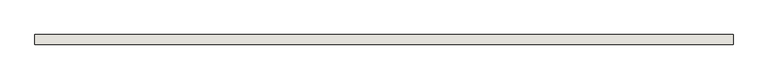
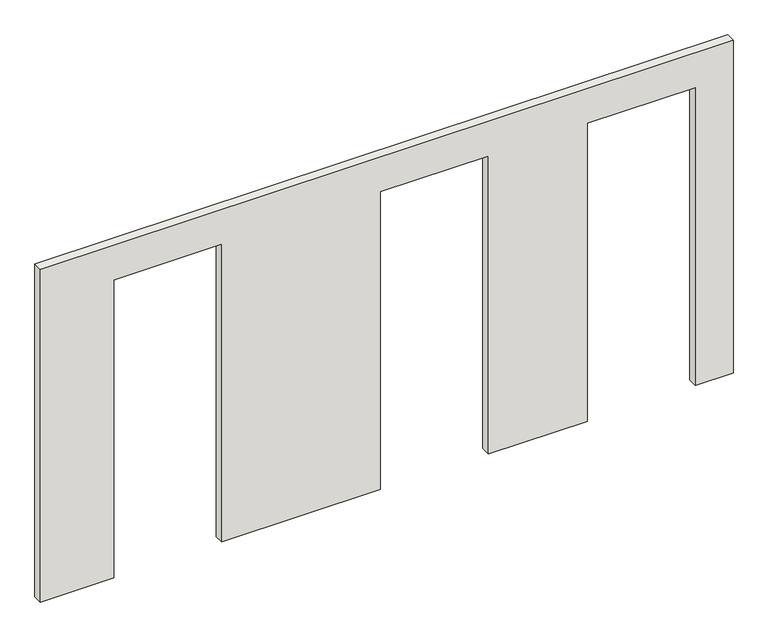
"""IFC4 building model written with IfcOpenShell, lengths in millimetres: wall geometry, 0_3d."""

import ifcopenshell
import ifcopenshell.guid

model = None  # the IFC model being written
_history = None  # IfcOwnerHistory: only IFC2X3 demands one
_inside = {}  # id of a spatial element -> (the spatial element, [elements in it])
_under = {}  # id of a project, library or spatial element -> (it, [spatial elements below it])
_declared = {}  # id of a project -> (the project, [libraries it declares])
_typed = {}  # id of a type object -> (the type object, [elements of that type])
_made_of = {}  # id of a material, layer set ... -> (it, [elements and type objects made of it])


def new_model(schema):
    """Start an empty IFC model of exactly this schema.

    Asked for "IFC4X3", IfcOpenShell would pick the latest addendum, in which some entities
    have other attributes; the version numbers below select the first issue.
    IFC2X3 requires an IfcOwnerHistory on every rooted entity: one is made here for all.
    """
    global model, _history
    if schema == "IFC4X3":
        model = ifcopenshell.file(schema_version=(4, 3, 0, 0))
    else:
        model = ifcopenshell.file(schema=schema)
    _inside.clear()
    _under.clear()
    _declared.clear()
    _typed.clear()
    _made_of.clear()
    _history = None
    if model.schema == "IFC2X3":
        org = make("IfcOrganization", Name="unknown")
        user = make(
            "IfcPersonAndOrganization",
            ThePerson=make("IfcPerson", FamilyName="unknown"),
            TheOrganization=org,
        )
        app = make(
            "IfcApplication",
            ApplicationDeveloper=org,
            Version="unknown",
            ApplicationFullName="unknown",
            ApplicationIdentifier="unknown",
        )
        _history = make(
            "IfcOwnerHistory",
            OwningUser=user,
            OwningApplication=app,
            ChangeAction="ADDED",
            CreationDate=0,
        )
    return model


def make(cls, **values):
    """One entity of the class cls with the attributes given. An attribute that is None is left unset."""
    return model.create_entity(
        cls, **{name: value for name, value in values.items() if value is not None}
    )


def rooted(cls, **values):
    """An entity with a GlobalId (a new one), such as an element, a storey or a relation."""
    return make(cls, GlobalId=ifcopenshell.guid.new(), OwnerHistory=_history, **values)


def si_unit(unit_type, name, prefix=None):
    """IfcSIUnit, for example si_unit("LENGTHUNIT", "METRE", prefix="MILLI")."""
    return make("IfcSIUnit", UnitType=unit_type, Prefix=prefix, Name=name)


def assignment(units):
    """IfcUnitAssignment: the units of a project."""
    return None if units is None else make("IfcUnitAssignment", Units=units)


def point(xyz):
    """IfcCartesianPoint."""
    return None if xyz is None else make("IfcCartesianPoint", Coordinates=xyz)


def direction(xyz):
    """IfcDirection."""
    return None if xyz is None else make("IfcDirection", DirectionRatios=xyz)


def frame(location, z_axis=None, x_axis=None):
    """IfcAxis2Placement3D, a coordinate frame: its origin and axes. An axis left out is left unset."""
    return make(
        "IfcAxis2Placement3D",
        Location=point(location),
        Axis=direction(z_axis),
        RefDirection=direction(x_axis),
    )


def origin():
    """The frame at (0, 0, 0) with its axes left unset."""
    return frame((0.0, 0.0, 0.0))


def place(relative_to, where):
    """IfcLocalPlacement: puts the frame where relative to a parent placement (None: the world)."""
    return make(
        "IfcLocalPlacement", PlacementRelTo=relative_to, RelativePlacement=where
    )


def context(
    kind, dimensions, precision=None, world=None, true_north=None, identifier=None
):
    """IfcGeometricRepresentationContext, for example the 3D "Model" context."""
    return make(
        "IfcGeometricRepresentationContext",
        ContextIdentifier=identifier,
        ContextType=kind,
        CoordinateSpaceDimension=dimensions,
        Precision=precision,
        WorldCoordinateSystem=world,
        TrueNorth=true_north,
    )


def project(units=None, contexts=None):
    """IfcProject with its units and contexts."""
    return rooted(
        "IfcProject",
        Name="project",
        RepresentationContexts=contexts,
        UnitsInContext=assignment(units),
    )


def spatial(cls, under=None, at=None, **own):
    """A site, building, storey or space (cls), placed at a placement, below another one or the project."""
    s = rooted(cls, ObjectPlacement=at, **own)
    if under is not None:
        _under.setdefault(under.id(), (under, []))[1].append(s)
    return s


def polyline(points):
    """IfcPolyline through the points."""
    return make("IfcPolyline", Points=[point(p) for p in points])


def outline(outer, holes=None, kind="AREA"):
    """IfcArbitraryClosedProfileDef: a profile drawn as a closed curve; with holes, ...WithVoids."""
    if holes is None:
        return make("IfcArbitraryClosedProfileDef", ProfileType=kind, OuterCurve=outer)
    return make(
        "IfcArbitraryProfileDefWithVoids",
        ProfileType=kind,
        OuterCurve=outer,
        InnerCurves=holes,
    )


def extrude(swept, where, along, depth):
    """IfcExtrudedAreaSolid: the profile swept, set in the frame where, extruded along a direction by depth."""
    return make(
        "IfcExtrudedAreaSolid",
        SweptArea=swept,
        Position=where,
        ExtrudedDirection=direction(along),
        Depth=depth,
    )


def shape(context_of_items, identifier, shape_type, items):
    """IfcShapeRepresentation: the items that make up one representation, for example the "Body"."""
    return make(
        "IfcShapeRepresentation",
        ContextOfItems=context_of_items,
        RepresentationIdentifier=identifier,
        RepresentationType=shape_type,
        Items=items,
    )


def source(mapping_origin, context_of_items, identifier, shape_type, items):
    """IfcRepresentationMap: a shape defined once, which mapped items show again and again."""
    return make(
        "IfcRepresentationMap",
        MappingOrigin=mapping_origin,
        MappedRepresentation=shape(context_of_items, identifier, shape_type, items),
    )


def transform(
    local_origin,
    x_axis=None,
    y_axis=None,
    z_axis=None,
    scale=None,
    scale2=None,
    scale3=None,
    uniform=True,
):
    """IfcCartesianTransformationOperator3D, or its non-uniform kind. x_axis, y_axis, z_axis: its Axis1, 2, 3."""
    if uniform:
        return make(
            "IfcCartesianTransformationOperator3D",
            Axis1=direction(x_axis),
            Axis2=direction(y_axis),
            LocalOrigin=point(local_origin),
            Scale=scale,
            Axis3=direction(z_axis),
        )
    return make(
        "IfcCartesianTransformationOperator3DnonUniform",
        Axis1=direction(x_axis),
        Axis2=direction(y_axis),
        LocalOrigin=point(local_origin),
        Scale=scale,
        Axis3=direction(z_axis),
        Scale2=scale2,
        Scale3=scale3,
    )


def mapped(mapping_source, mapping_target):
    """IfcMappedItem: shows the shape of a source again, moved by a transform."""
    return make(
        "IfcMappedItem", MappingSource=mapping_source, MappingTarget=mapping_target
    )


def made_of(thing, what):
    """Note that an element or type object is made of a material, layer set ...; save() writes the relation."""
    if what is not None:
        _made_of.setdefault(what.id(), (what, []))[1].append(thing)
    return thing


def element(
    cls,
    number,
    at=None,
    inside=None,
    cuts=None,
    type_object=None,
    material=None,
    context=None,
    identifier="Body",
    shape_type=None,
    held_by="IfcProductDefinitionShape",
    body=None,
    shapes=None,
    **own,
):
    """One element of the class cls, such as IfcWall. Its Tag is "e" and its number.

    at: its placement. inside: the storey or other place that contains it. cuts: it is an
    opening in that element (IfcRelVoidsElement). A single representation is given by context,
    identifier, shape_type and body (its items); several are given by shapes. held_by: the class
    of the entity that holds the representations. save() writes the other relations.
    """
    e = rooted(cls, Tag="e%d" % number, ObjectPlacement=at, **own)
    if body is not None:
        shapes = [shape(context, identifier, shape_type, body)]
    if shapes is not None:
        e.Representation = make(held_by, Representations=shapes)
    if inside is not None:
        _inside.setdefault(inside.id(), (inside, []))[1].append(e)
    if cuts is not None:
        rooted(
            "IfcRelVoidsElement", RelatingBuildingElement=cuts, RelatedOpeningElement=e
        )
    if type_object is not None:
        _typed.setdefault(type_object.id(), (type_object, []))[1].append(e)
    return made_of(e, material)


def aggregate(whole, parts):
    """IfcRelAggregates: a whole, such as a stair, and the parts it consists of."""
    return rooted("IfcRelAggregates", RelatingObject=whole, RelatedObjects=parts)


def save(model, path):
    """Write the relations noted so far, then the file.

    IfcRelAggregates (storeys below a building ...), IfcRelContainedInSpatialStructure (elements
    in a storey), IfcRelDefinesByType, IfcRelAssociatesMaterial and IfcRelDeclares: one each for
    every whole, place, type object, material and project.
    """
    for whole, parts in _under.values():
        aggregate(whole, parts)
    for where, things in _inside.values():
        rooted(
            "IfcRelContainedInSpatialStructure",
            RelatedElements=things,
            RelatingStructure=where,
        )
    for kind, things in _typed.values():
        rooted("IfcRelDefinesByType", RelatedObjects=things, RelatingType=kind)
    for what, things in _made_of.values():
        rooted("IfcRelAssociatesMaterial", RelatedObjects=things, RelatingMaterial=what)
    for by, libraries in _declared.values():
        rooted("IfcRelDeclares", RelatingContext=by, RelatedDefinitions=libraries)
    model.write(path)


def wall_c889103b(model_context):
    return source(origin(), model_context, "Body", "SweptSolid", [
        extrude(outline(polyline([(0.0, 4475.0), (2580.0, 4475.0), (2580.0, 5360.0), (0.0, 5360.0), (0.0, 5670.0), (2880.0, 5670.0), (2880.0, 0.0), (0.0, 0.0), (0.0, 600.0), (2580.0, 600.0), (2580.0, 1485.0), (0.0, 1485.0), (0.0, 2782.7134747), (2580.0, 2782.7134747), (2580.0, 3667.7134747), (0.0, 3667.7134747), (0.0, 4475.0)])), frame((0.0, 0.0, 0.0), z_axis=(0.0, 1.0, 0.0), x_axis=(0.0, 0.0, 1.0)), (0.0, 0.0, 1.0), 78.0),
    ])


if __name__ == "__main__":
    model = new_model("IFC4")
    model_context = context("Model", 3, world=origin())
    ifc_project = project(units=[si_unit("LENGTHUNIT", "METRE", prefix="MILLI")], contexts=[model_context])
    site = spatial("IfcSite", under=ifc_project)
    building = spatial("IfcBuilding", under=site)
    placement = place(None, origin())
    wall_shape = wall_c889103b(model_context)
    element("IfcWall", 1, ObjectType="0_3d", at=placement, inside=building, context=model_context, shape_type="MappedRepresentation", body=[
        mapped(wall_shape, transform((0.0, 0.0, 0.0), x_axis=(1.0, 0.0, 0.0), y_axis=(0.0, 1.0, 0.0), z_axis=(0.0, 0.0, 1.0))),
    ])
    save(model, "model.ifc")

# Revit data of these elements
# Element 1 (IfcWall, "0_3d")
#   Materials on its faces: "glas"
# Materials
#   "glas": class "Unassigned", colour RGB 250 253 254, transparency 0.95
